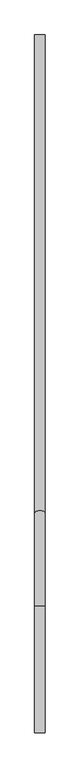
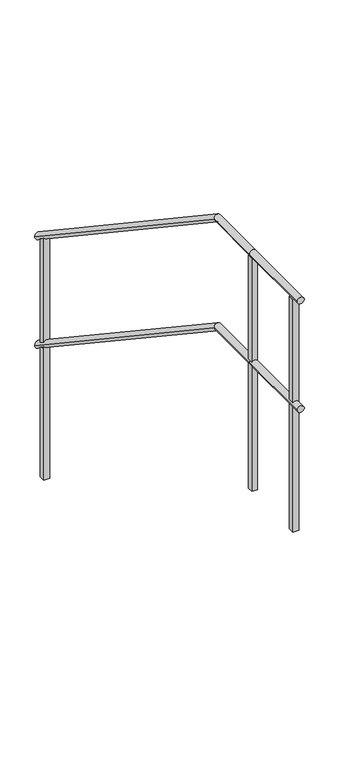
"""IFC4 building model written with IfcOpenShell, lengths in millimetres: railing geometry."""

from ifc_helpers import new_model, si_unit, frame, origin, place, context, project, spatial, polyline, circle_curve, ellipse_curve, outline, extrude, source, transform, mapped, element, save
from ifc_brep_helpers import plane_surface, cylinder_surface, advanced_brep


def railing_4ec7f6e5(model_context):
    return source(origin(), model_context, "Body", "SolidModel", [
        advanced_brep(
        [(13536.7845799, 439.5208589, 9334.9618634), (13566.7845799, 439.5208589, 9334.9618634), (13536.7845799, 799.5208589, 9334.9618634), (13566.7845799, 799.5208589, 9334.9618634)],
        [
            (0, 1, circle_curve(frame((13551.7845799, 439.5208589, 9334.9618634), z_axis=(0.0, -1.0, 0.0), x_axis=(1.0, 0.0, 0.0)), 15.0)),
            (1, 0, circle_curve(frame((13551.7845799, 439.5208589, 9334.9618634), z_axis=(0.0, -1.0, 0.0), x_axis=(1.0, 0.0, 0.0)), 15.0)),
            (2, 3, circle_curve(frame((13551.7845799, 799.5208589, 9334.9618634), z_axis=(0.0, 1.0, 0.0), x_axis=(1.0, 0.0, 0.0)), 15.0)),
            (3, 2, circle_curve(frame((13551.7845799, 799.5208589, 9334.9618634), z_axis=(0.0, 1.0, 0.0), x_axis=(1.0, 0.0, 0.0)), 15.0)),
            (0, 2),
            (3, 1),
        ],
        [
            plane_surface(frame((13551.7845799, 439.5208589, 9349.9618634), z_axis=(0.0, -1.0, 0.0), x_axis=(0.0, 0.0, 1.0))),
            plane_surface(frame((13551.7845799, 799.5208589, 9349.9618634), z_axis=(0.0, 1.0, 0.0), x_axis=(0.0, 0.0, 1.0))),
            cylinder_surface(frame((13551.7845799, 439.5208589, 9334.9618634), z_axis=(0.0, -1.0, 0.0), x_axis=(1.0, 0.0, 0.0)), 15.0),
        ],
        [
            (0, [[1, 2]]),
            (1, [[3, 4]]),
            (2, [[-1, 5, -4, 6]]),
            (2, [[-2, -6, -3, -5]]),
        ],
    ),
        advanced_brep(
        [(13536.7845799, 799.5208589, 9334.9618634), (13566.7845799, 799.5208589, 9334.9618634), (13536.7845799, 1064.9792243, 9334.9618634), (13566.7845799, 1064.9792243, 9334.9618634), (13536.7845799, 2419.5208589, 8431.934107), (13566.7845799, 2419.5208589, 8431.934107)],
        [
            (0, 1, circle_curve(frame((13551.7845799, 799.5208589, 9334.9618634), z_axis=(0.0, -1.0, 0.0), x_axis=(1.0, 0.0, 0.0)), 15.0)),
            (1, 0, circle_curve(frame((13551.7845799, 799.5208589, 9334.9618634), z_axis=(0.0, -1.0, 0.0), x_axis=(1.0, 0.0, 0.0)), 15.0)),
            (0, 2),
            (2, 3, ellipse_curve(frame((13551.7845799, 1064.9792243, 9334.9618634), z_axis=(0.0, -0.9570920264890528, 0.28978414868843017), x_axis=(0.0, -0.2897841486884305, -0.9570920264890528)), 15.6724741, 15.0)),
            (3, 1),
            (3, 2, ellipse_curve(frame((13551.7845799, 1064.9792243, 9334.9618634), z_axis=(0.0, -0.9570920264890528, 0.28978414868843017), x_axis=(0.0, -0.2897841486884305, -0.9570920264890528)), 15.6724741, 15.0)),
            (4, 5, ellipse_curve(frame((13551.7845799, 2419.5208589, 8431.934107), z_axis=(0.0, 1.0, 0.0), x_axis=(0.0, 0.0, 1.0)), 18.0277564, 15.0)),
            (5, 4, ellipse_curve(frame((13551.7845799, 2419.5208589, 8431.934107), z_axis=(0.0, 1.0, 0.0), x_axis=(0.0, 0.0, 1.0)), 18.0277564, 15.0)),
            (2, 4),
            (5, 3),
        ],
        [
            plane_surface(frame((13551.7845799, 799.5208589, 9349.9618634), z_axis=(0.0, -1.0, 0.0), x_axis=(0.0, 0.0, 1.0))),
            cylinder_surface(frame((13551.7845799, 799.5208589, 9334.9618634), z_axis=(0.0, -1.0, 0.0), x_axis=(1.0, 0.0, 0.0)), 15.0),
            plane_surface(frame((13551.7845799, 2419.5208589, 8449.9618634), z_axis=(0.0, 1.0, 0.0), x_axis=(0.0, 0.0, 1.0))),
            cylinder_surface(frame((13551.7845799, 1061.2003559, 9337.481109), z_axis=(0.0, -0.8320502943378436, 0.5547001962252293), x_axis=(1.0, 0.0, 0.0)), 15.0),
        ],
        [
            (0, [[1, 2]]),
            (1, [[-1, 3, 4, 5]]),
            (1, [[-2, -5, 6, -3]]),
            (2, [[7, 8]]),
            (3, [[-4, 9, -8, 10]]),
            (3, [[-6, -10, -7, -9]]),
        ],
    ),
        advanced_brep(
        [(13536.7845799, 439.5208589, 9834.9618634), (13566.7845799, 439.5208589, 9834.9618634), (13536.7845799, 799.5208589, 9834.9618634), (13566.7845799, 799.5208589, 9834.9618634)],
        [
            (0, 1, circle_curve(frame((13551.7845799, 439.5208589, 9834.9618634), z_axis=(0.0, -1.0, 0.0), x_axis=(1.0, 0.0, 0.0)), 15.0)),
            (1, 0, circle_curve(frame((13551.7845799, 439.5208589, 9834.9618634), z_axis=(0.0, -1.0, 0.0), x_axis=(1.0, 0.0, 0.0)), 15.0)),
            (2, 3, circle_curve(frame((13551.7845799, 799.5208589, 9834.9618634), z_axis=(0.0, 1.0, 0.0), x_axis=(1.0, 0.0, 0.0)), 15.0)),
            (3, 2, circle_curve(frame((13551.7845799, 799.5208589, 9834.9618634), z_axis=(0.0, 1.0, 0.0), x_axis=(1.0, 0.0, 0.0)), 15.0)),
            (0, 2),
            (3, 1),
        ],
        [
            plane_surface(frame((13551.7845799, 439.5208589, 9849.9618634), z_axis=(0.0, -1.0, 0.0), x_axis=(0.0, 0.0, 1.0))),
            plane_surface(frame((13551.7845799, 799.5208589, 9849.9618634), z_axis=(0.0, 1.0, 0.0), x_axis=(0.0, 0.0, 1.0))),
            cylinder_surface(frame((13551.7845799, 439.5208589, 9834.9618634), z_axis=(0.0, -1.0, 0.0), x_axis=(1.0, 0.0, 0.0)), 15.0),
        ],
        [
            (0, [[1, 2]]),
            (1, [[3, 4]]),
            (2, [[-1, 5, -4, 6]]),
            (2, [[-2, -6, -3, -5]]),
        ],
    ),
        advanced_brep(
        [(13536.7845799, 799.5208589, 9834.9618634), (13566.7845799, 799.5208589, 9834.9618634), (13536.7845799, 1064.9792243, 9834.9618634), (13566.7845799, 1064.9792243, 9834.9618634), (13536.7845799, 2419.5208589, 8931.934107), (13566.7845799, 2419.5208589, 8931.934107)],
        [
            (0, 1, circle_curve(frame((13551.7845799, 799.5208589, 9834.9618634), z_axis=(0.0, -1.0, 0.0), x_axis=(1.0, 0.0, 0.0)), 15.0)),
            (1, 0, circle_curve(frame((13551.7845799, 799.5208589, 9834.9618634), z_axis=(0.0, -1.0, 0.0), x_axis=(1.0, 0.0, 0.0)), 15.0)),
            (0, 2),
            (2, 3, ellipse_curve(frame((13551.7845799, 1064.9792243, 9834.9618634), z_axis=(0.0, -0.9570920264890528, 0.28978414868843017), x_axis=(0.0, -0.2897841486884305, -0.9570920264890528)), 15.6724741, 15.0)),
            (3, 1),
            (3, 2, ellipse_curve(frame((13551.7845799, 1064.9792243, 9834.9618634), z_axis=(0.0, -0.9570920264890528, 0.28978414868843017), x_axis=(0.0, -0.2897841486884305, -0.9570920264890528)), 15.6724741, 15.0)),
            (4, 5, ellipse_curve(frame((13551.7845799, 2419.5208589, 8931.934107), z_axis=(0.0, 1.0, 0.0), x_axis=(0.0, 0.0, 1.0)), 18.0277564, 15.0)),
            (5, 4, ellipse_curve(frame((13551.7845799, 2419.5208589, 8931.934107), z_axis=(0.0, 1.0, 0.0), x_axis=(0.0, 0.0, 1.0)), 18.0277564, 15.0)),
            (2, 4),
            (5, 3),
        ],
        [
            plane_surface(frame((13551.7845799, 799.5208589, 9849.9618634), z_axis=(0.0, -1.0, 0.0), x_axis=(0.0, 0.0, 1.0))),
            cylinder_surface(frame((13551.7845799, 799.5208589, 9834.9618634), z_axis=(0.0, -1.0, 0.0), x_axis=(1.0, 0.0, 0.0)), 15.0),
            plane_surface(frame((13551.7845799, 2419.5208589, 8949.9618634), z_axis=(0.0, 1.0, 0.0), x_axis=(0.0, 0.0, 1.0))),
            cylinder_surface(frame((13551.7845799, 1061.2003559, 9837.481109), z_axis=(0.0, -0.8320502943378436, 0.5547001962252293), x_axis=(1.0, 0.0, 0.0)), 15.0),
        ],
        [
            (0, [[1, 2]]),
            (1, [[-1, 3, 4, 5]]),
            (1, [[-2, -5, 6, -3]]),
            (2, [[7, 8]]),
            (3, [[-4, 9, -8, 10]]),
            (3, [[-6, -10, -7, -9]]),
        ],
    ),
        extrude(outline(polyline([(13564.2845799, 787.0208589), (13539.2845799, 787.0208589), (13539.2845799, 812.0208589), (13564.2845799, 812.0208589), (13564.2845799, 787.0208589)])), frame((0.0, 0.0, 8749.9618634), z_axis=(0.0, 0.0, 1.0), x_axis=(1.0, 0.0, 0.0)), (0.0, 0.0, 1.0), 1070.0),
        extrude(outline(polyline([(2357.0208589, 7849.9618634), (2357.0208589, 8961.62853), (2382.0208589, 8944.9618634), (2382.0208589, 7849.9618634), (2357.0208589, 7849.9618634)])), frame((13539.2845799, 0.0, 0.0), z_axis=(1.0, 0.0, 0.0), x_axis=(0.0, 1.0, 0.0)), (0.0, 0.0, 1.0), 25.0),
        extrude(outline(polyline([(13564.2845799, 477.0208589), (13539.2845799, 477.0208589), (13539.2845799, 502.0208589), (13564.2845799, 502.0208589), (13564.2845799, 477.0208589)])), frame((0.0, 0.0, 8749.9618634), z_axis=(0.0, 0.0, 1.0), x_axis=(1.0, 0.0, 0.0)), (0.0, 0.0, 1.0), 1070.0),
    ])


if __name__ == "__main__":
    model = new_model("IFC4")
    model_context = context("Model", 3, world=origin())
    ifc_project = project(units=[si_unit("LENGTHUNIT", "METRE", prefix="MILLI")], contexts=[model_context])
    site = spatial("IfcSite", under=ifc_project)
    building = spatial("IfcBuilding", under=site)
    placement = place(None, origin())
    railing_shape = railing_4ec7f6e5(model_context)
    element("IfcRailing", 1, at=placement, inside=building, context=model_context, shape_type="MappedRepresentation", body=[
        mapped(railing_shape, transform((0.0, 0.0, 0.0), x_axis=(1.0, 0.0, 0.0), y_axis=(0.0, 1.0, 0.0), z_axis=(0.0, 0.0, 1.0))),
    ])
    save(model, "model.ifc")
